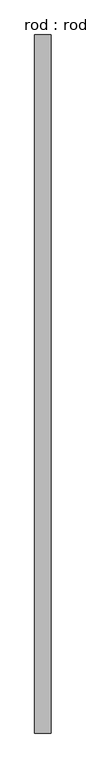
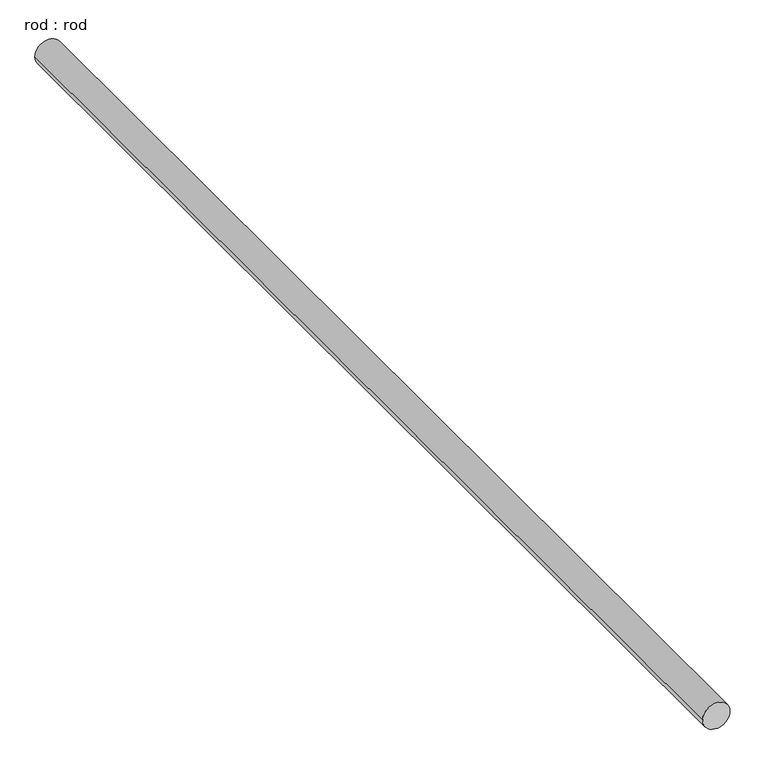
"""IFC4 building model written with IfcOpenShell, lengths in millimetres: proxy geometry, rod : rod."""

from ifc_helpers import new_model, si_unit, point, frame, frame_2d, origin, place, context, project, spatial, circle_curve, trimmed, segment, composite_curve, outline, extrude, source, transform, mapped, element, save


def rod_rod_2f618551(model_context):
    return source(origin(), model_context, "Body", "SweptSolid", [
        extrude(outline(composite_curve([segment(trimmed(circle_curve(frame_2d((0.0108462, 0.0)), 200.0), [point((0.0108462, 200.0))], [point((0.0108462, -200.0))], False, "CARTESIAN"), True, "CONTINUOUS"), segment(trimmed(circle_curve(frame_2d((0.0108462, 0.0)), 200.0), [point((0.0108462, -200.0))], [point((0.0108462, 200.0))], False, "CARTESIAN"), True, "CONTINUOUS")], self_intersect=False)), frame((0.0, -4389.5861498, 0.0), z_axis=(0.0, 1.0, 0.0), x_axis=(0.0, 0.0, 1.0)), (0.0, 0.0, 1.0), 16964.6295304),
    ])


if __name__ == "__main__":
    model = new_model("IFC4")
    model_context = context("Model", 3, world=origin())
    ifc_project = project(units=[si_unit("LENGTHUNIT", "METRE", prefix="MILLI")], contexts=[model_context])
    site = spatial("IfcSite", under=ifc_project)
    building = spatial("IfcBuilding", under=site)
    placement = place(None, origin())
    rod_rod_shape = rod_rod_2f618551(model_context)
    element("IfcBuildingElementProxy", 1, Name="rod : rod", ObjectType="rod : rod", at=placement, inside=building, context=model_context, shape_type="MappedRepresentation", body=[
        mapped(rod_rod_shape, transform((0.0, 0.0, 0.0), x_axis=(1.0, 0.0, 0.0), y_axis=(0.0, 1.0, 0.0), z_axis=(0.0, 0.0, 1.0))),
    ])
    save(model, "model.ifc")

# Revit data of these elements
# Type "rod : rod"
#   Default Elevation = 0
